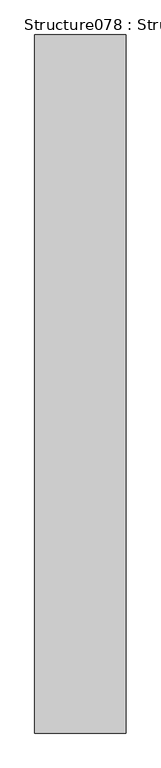
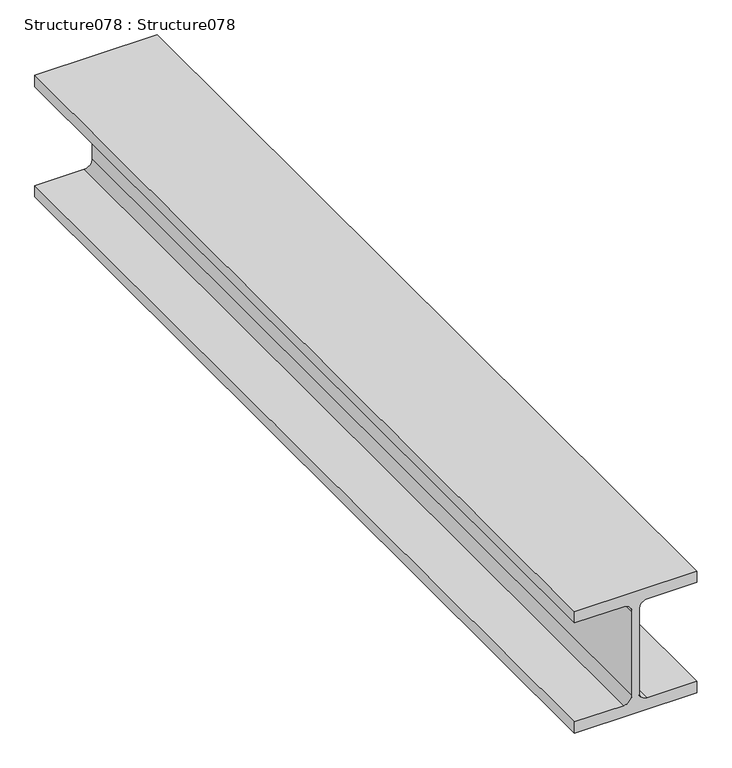
"""IFC4 building model written with IfcOpenShell, lengths in millimetres: proxy geometry, Structure078 : Structure078."""

from ifc_helpers import new_model, si_unit, point, frame, frame_2d, origin, place, context, project, spatial, polyline, circle_curve, trimmed, segment, composite_curve, outline, extrude, source, transform, mapped, element, save


def structure078_structure078_99db3ef5(model_context):
    return source(origin(), model_context, "Body", "SweptSolid", [
        extrude(outline(composite_curve([segment(trimmed(circle_curve(frame_2d((36399.5335, -2417.5018494)), 17.7165), [point((36399.5335, -2435.2183494))], [point((36417.25, -2417.5018494))], True, "CARTESIAN"), True, "CONTINUOUS"), segment(polyline([(36417.25, -2417.5018494), (36417.25, -2312.0918494), (36442.396, -2312.0918494), (36442.396, -2573.7118494), (36417.25, -2573.7118494), (36417.25, -2468.3018494)]), True, "CONTINUOUS"), segment(trimmed(circle_curve(frame_2d((36399.5335, -2468.3018494)), 17.7165), [point((36417.25, -2468.3018494))], [point((36399.5335, -2450.5853494))], True, "CARTESIAN"), True, "CONTINUOUS"), segment(polyline([(36399.5335, -2450.5853494), (36210.9385, -2450.5853494)]), True, "CONTINUOUS"), segment(trimmed(circle_curve(frame_2d((36210.9385, -2468.3018494)), 17.7165), [point((36210.9385, -2450.5853494))], [point((36193.222, -2468.3018494))], True, "CARTESIAN"), True, "CONTINUOUS"), segment(polyline([(36193.222, -2468.3018494), (36193.222, -2573.7118494), (36168.076, -2573.7118494), (36168.076, -2312.0918494), (36193.222, -2312.0918494), (36193.222, -2417.5018494)]), True, "CONTINUOUS"), segment(trimmed(circle_curve(frame_2d((36210.9385, -2417.5018494)), 17.7165), [point((36193.222, -2417.5018494))], [point((36210.9385, -2435.2183494))], True, "CARTESIAN"), True, "CONTINUOUS"), segment(polyline([(36210.9385, -2435.2183494), (36399.5335, -2435.2183494)]), True, "CONTINUOUS")], self_intersect=False)), frame((0.0, 998.1548221, 0.0), z_axis=(0.0, 1.0, 0.0), x_axis=(0.0, 0.0, 1.0)), (0.0, 0.0, 1.0), 2000.0),
    ])


if __name__ == "__main__":
    model = new_model("IFC4")
    model_context = context("Model", 3, world=origin())
    ifc_project = project(units=[si_unit("LENGTHUNIT", "METRE", prefix="MILLI")], contexts=[model_context])
    site = spatial("IfcSite", under=ifc_project)
    building = spatial("IfcBuilding", under=site)
    placement = place(None, origin())
    structure078_structure078_shape = structure078_structure078_99db3ef5(model_context)
    element("IfcBuildingElementProxy", 1, Name="Structure078 : Structure078", ObjectType="Structure078 : Structure078", at=placement, inside=building, context=model_context, shape_type="MappedRepresentation", body=[
        mapped(structure078_structure078_shape, transform((0.0, 0.0, 0.0), x_axis=(1.0, 0.0, 0.0), y_axis=(0.0, 1.0, 0.0), z_axis=(0.0, 0.0, 1.0))),
    ])
    save(model, "model.ifc")

# Revit data of these elements
# Type "Structure078 : Structure078"
#   NameOverride = "Structure078"
# Element 1 (IfcBuildingElementProxy, "Structure078 : Structure078")
#   Materials on its faces: "STEEL STRUCTURE (SEE STRUCTURAL DWGS)"
# Materials
#   "STEEL STRUCTURE (SEE STRUCTURAL DWGS)": class "Unassigned", colour RGB 128 128 128, transparency 0, Cost = 0
